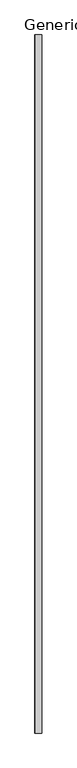
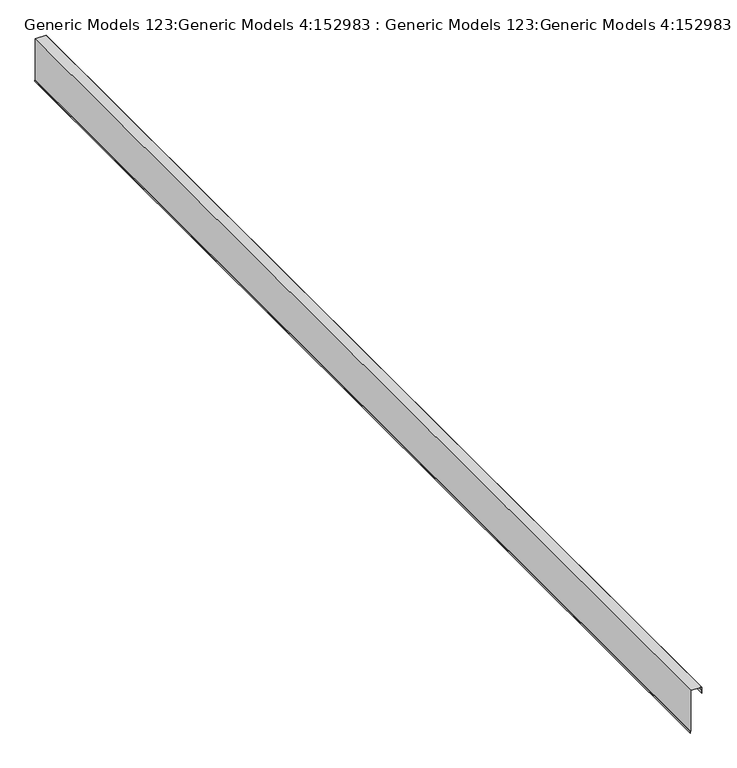
"""IFC4 building model written with IfcOpenShell, lengths in millimetres: proxy geometry, Generic Models 123:Generic Models 4:152983 : Generic Models 123:Generic Models 4:152983."""

from ifc_helpers import new_model, si_unit, frame, origin, place, context, project, spatial, polyline, outline, extrude, source, transform, mapped, element, save


def generic_models_123_generic_models_4_152983_generic_models_189d41ed(model_context):
    return source(origin(), model_context, "Body", "SweptSolid", [
        extrude(outline(polyline([(3722.7610194, 7238.4813381), (3715.6290789, 7241.0771521), (3676.3784351, 7241.0771521), (3676.3784351, 7241.8709021), (3715.7690384, 7241.8709021), (3722.900979, 7239.2750881), (3781.2294539, 7239.2750881), (3788.875361, 7055.7733174), (3075.0790007, 7055.7733174), (3066.1660646, 7052.529274), (3047.1435521, 7052.529274), (3047.1435521, 7053.323024), (3066.0261051, 7053.323024), (3074.9390411, 7056.5670674), (3788.0478493, 7056.5670674), (3780.4680881, 7238.4813381), (3722.7610194, 7238.4813381)])), frame((0.0, -6674.7974793, 0.0), z_axis=(0.0, 1.0, 0.0), x_axis=(0.0, 0.0, 1.0)), (0.0, 0.0, 1.0), 18643.6),
    ])


if __name__ == "__main__":
    model = new_model("IFC4")
    model_context = context("Model", 3, world=origin())
    ifc_project = project(units=[si_unit("LENGTHUNIT", "METRE", prefix="MILLI")], contexts=[model_context])
    site = spatial("IfcSite", under=ifc_project)
    building = spatial("IfcBuilding", under=site)
    placement = place(None, origin())
    generic_models_123_generic_models_4_152983_generic_models_shape = generic_models_123_generic_models_4_152983_generic_models_189d41ed(model_context)
    element("IfcBuildingElementProxy", 1, Name="Generic Models 123:Generic Models 4:152983 : Generic Models 123:Generic Models 4:152983", ObjectType="Generic Models 123:Generic Models 4:152983 : Generic Models 123:Generic Models 4:152983", at=placement, inside=building, context=model_context, shape_type="MappedRepresentation", body=[
        mapped(generic_models_123_generic_models_4_152983_generic_models_shape, transform((0.0, 0.0, 0.0), x_axis=(1.0, 0.0, 0.0), y_axis=(0.0, 1.0, 0.0), z_axis=(0.0, 0.0, 1.0))),
    ])
    save(model, "model.ifc")

# Revit data of these elements
# Type "Generic Models 123:Generic Models 4:152983 : Generic Models 123:Generic Models 4:152983"
#   NameOverride = "Generic Models 123:Generic Models 4:152983"
#   ObjectTypeOverride = "Generic Models 123:Generic Models 4"
#   Reference = "Generic Models 4"
#   Category = "Generic Models"
#   Tag = "152983"
# Element 1 (IfcBuildingElementProxy, "Generic Models 123:Generic Models 4:152983 : Generic Models 123:Generic Models 4:152983")
#   Materials on its faces: "_(2) LAYERS NO. 30 ASTM D226 ASPHALT SATURATED ORGANIC FELT 997"
# Materials
#   "_(2) LAYERS NO. 30 ASTM D226 ASPHALT SATURATED ORGANIC FELT 997": class "Unassigned", colour RGB 67 154 161, transparency 0
